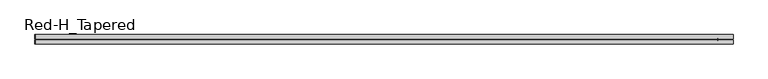
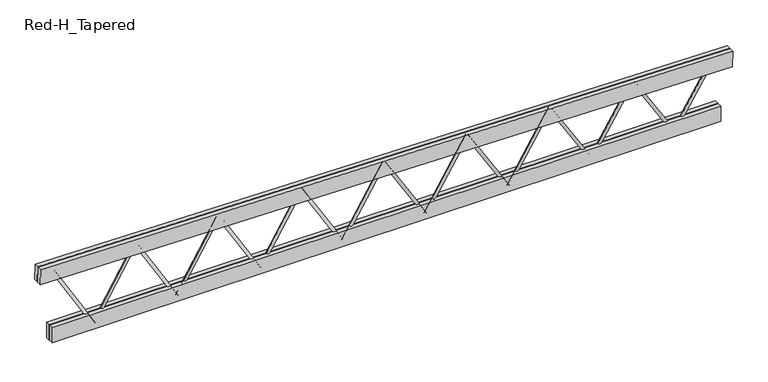
"""IFC4 building model written with IfcOpenShell, lengths in millimetres: beam geometry, Construction_Frames_RedBuilt_Openweb_Red-H_Tapered : Red-H_Tapered."""

from ifc_helpers import new_model, si_unit, point, frame, origin, origin_2d, place, context, project, spatial, polyline, circle_curve, trimmed, segment, composite_curve, outline, extrude, source, transform, mapped, element, save


def red_h_tapered_b0e51fd6(model_context):
    return source(origin(), model_context, "Body", "SweptSolid", [
        extrude(outline(composite_curve([segment(trimmed(circle_curve(origin_2d(), 12.7), [point((0.0, 12.7000001))], [point((0.0, -12.7))], False, "CARTESIAN"), True, "CONTINUOUS"), segment(trimmed(circle_curve(origin_2d(), 12.7), [point((0.0, -12.7))], [point((0.0, 12.7000001))], False, "CARTESIAN"), True, "CONTINUOUS")], self_intersect=False)), frame((2530.5740404, 0.0, -367.0101562), z_axis=(0.5262103953903533, 0.0, 0.8503544083399157), x_axis=(0.0, -1.0, 0.0)), (0.0, 0.0, 1.0), 687.0076691),
        extrude(outline(composite_curve([segment(trimmed(circle_curve(origin_2d(), 12.7), [point((0.0, -12.7))], [point((0.0, 12.7))], False, "CARTESIAN"), True, "CONTINUOUS"), segment(trimmed(circle_curve(origin_2d(), 12.7), [point((0.0, 12.7))], [point((0.0, -12.7))], False, "CARTESIAN"), True, "CONTINUOUS")], self_intersect=False)), frame((2530.5740404, 0.0, -367.0101562), z_axis=(-0.5236364879758304, 0.0, 0.8519417987517328), x_axis=(0.0, -1.0, 0.0)), (0.0, 0.0, 1.0), 690.3846189),
        extrude(outline(composite_curve([segment(trimmed(circle_curve(origin_2d(), 12.7), [point((0.0, 12.7))], [point((0.0, -12.6999999))], False, "CARTESIAN"), True, "CONTINUOUS"), segment(trimmed(circle_curve(origin_2d(), 12.7), [point((0.0, -12.6999999))], [point((0.0, 12.7))], False, "CARTESIAN"), True, "CONTINUOUS")], self_intersect=False)), frame((1807.552886, 0.0, -367.0101562), z_axis=(0.5236364879758294, 0.0, 0.8519417987517335), x_axis=(0.0, -1.0, 0.0)), (0.0, 0.0, 1.0), 690.3846189),
        extrude(outline(composite_curve([segment(trimmed(circle_curve(origin_2d(), 12.7), [point((0.0, -12.7))], [point((0.0, 12.7))], False, "CARTESIAN"), True, "CONTINUOUS"), segment(trimmed(circle_curve(origin_2d(), 12.7), [point((0.0, 12.7))], [point((0.0, -12.7))], False, "CARTESIAN"), True, "CONTINUOUS")], self_intersect=False)), frame((1807.552886, 0.0, -367.0101562), z_axis=(-0.5210829422122787, 0.0, 0.8535060441118124), x_axis=(0.0, -1.0, 0.0)), (0.0, 0.0, 1.0), 693.7678207),
        extrude(outline(composite_curve([segment(trimmed(circle_curve(origin_2d(), 12.7), [point((0.0, 12.7000001))], [point((0.0, -12.6999999))], False, "CARTESIAN"), True, "CONTINUOUS"), segment(trimmed(circle_curve(origin_2d(), 12.7), [point((0.0, -12.6999999))], [point((0.0, 12.7000001))], False, "CARTESIAN"), True, "CONTINUOUS")], self_intersect=False)), frame((1084.5317316, 0.0, -367.0101562), z_axis=(0.5210829422122776, 0.0, 0.8535060441118131), x_axis=(0.0, -1.0, 0.0)), (0.0, 0.0, 1.0), 693.7678207),
        extrude(outline(composite_curve([segment(trimmed(circle_curve(origin_2d(), 12.7), [point((0.0, -12.7))], [point((0.0, 12.7))], False, "CARTESIAN"), True, "CONTINUOUS"), segment(trimmed(circle_curve(origin_2d(), 12.7), [point((0.0, 12.7))], [point((0.0, -12.7))], False, "CARTESIAN"), True, "CONTINUOUS")], self_intersect=False)), frame((1084.5317316, 0.0, -367.0101562), z_axis=(-0.5185495980628914, 0.0, 0.855047550928493), x_axis=(0.0, -1.0, 0.0)), (0.0, 0.0, 1.0), 697.1571833),
        extrude(outline(composite_curve([segment(trimmed(circle_curve(origin_2d(), 12.7), [point((0.0, 12.7))], [point((0.0, -12.7))], False, "CARTESIAN"), True, "CONTINUOUS"), segment(trimmed(circle_curve(origin_2d(), 12.7), [point((0.0, -12.7))], [point((0.0, 12.7))], False, "CARTESIAN"), True, "CONTINUOUS")], self_intersect=False)), frame((361.5105772, 0.0, -367.0101562), z_axis=(0.5185495980628919, 0.0, 0.8550475509284927), x_axis=(0.0, -1.0, 0.0)), (0.0, 0.0, 1.0), 697.1571833),
        extrude(outline(composite_curve([segment(trimmed(circle_curve(origin_2d(), 12.7), [point((0.0, -12.7))], [point((0.0, 12.7))], False, "CARTESIAN"), True, "CONTINUOUS"), segment(trimmed(circle_curve(origin_2d(), 12.7), [point((0.0, 12.7))], [point((0.0, -12.7))], False, "CARTESIAN"), True, "CONTINUOUS")], self_intersect=False)), frame((361.5105772, 0.0, -367.0101562), z_axis=(-0.5160362950207581, 0.0, 0.8565667179042443), x_axis=(0.0, -1.0, 0.0)), (0.0, 0.0, 1.0), 700.5526175),
        extrude(outline(composite_curve([segment(trimmed(circle_curve(origin_2d(), 12.7), [point((0.0, -12.7))], [point((0.0, 12.7))], False, "CARTESIAN"), True, "CONTINUOUS"), segment(trimmed(circle_curve(origin_2d(), 12.7), [point((0.0, 12.7))], [point((0.0, -12.7))], False, "CARTESIAN"), True, "CONTINUOUS")], self_intersect=False)), frame((-361.5105772, 0.0, -367.0101562), z_axis=(0.5160362950207268, 0.0, 0.8565667179042632), x_axis=(0.0, -1.0, 0.0)), (0.0, 0.0, 1.0), 700.5526175),
        extrude(outline(composite_curve([segment(trimmed(circle_curve(origin_2d(), 12.7), [point((0.0, 12.7))], [point((0.0, -12.7))], False, "CARTESIAN"), True, "CONTINUOUS"), segment(trimmed(circle_curve(origin_2d(), 12.7), [point((0.0, -12.7))], [point((0.0, 12.7))], False, "CARTESIAN"), True, "CONTINUOUS")], self_intersect=False)), frame((-361.5105772, 0.0, -367.0101562), z_axis=(-0.5135428722107241, 0.0, 0.8580639360802667), x_axis=(0.0, -1.0, 0.0)), (0.0, 0.0, 1.0), 703.9540353),
        extrude(outline(composite_curve([segment(trimmed(circle_curve(origin_2d(), 12.7), [point((0.0, -12.7))], [point((0.0, 12.7))], False, "CARTESIAN"), True, "CONTINUOUS"), segment(trimmed(circle_curve(origin_2d(), 12.7), [point((0.0, 12.7))], [point((0.0, -12.7))], False, "CARTESIAN"), True, "CONTINUOUS")], self_intersect=False)), frame((-1084.5317316, 0.0, -367.0101562), z_axis=(0.5135428722107226, 0.0, 0.8580639360802675), x_axis=(0.0, -1.0, 0.0)), (0.0, 0.0, 1.0), 703.9540353),
        extrude(outline(composite_curve([segment(trimmed(circle_curve(origin_2d(), 12.7), [point((0.0, 12.7))], [point((0.0, -12.7))], False, "CARTESIAN"), True, "CONTINUOUS"), segment(trimmed(circle_curve(origin_2d(), 12.7), [point((0.0, -12.7))], [point((0.0, 12.7))], False, "CARTESIAN"), True, "CONTINUOUS")], self_intersect=False)), frame((-1084.5317316, 0.0, -367.0101562), z_axis=(-0.5110691684864845, 0.0, 0.8595395889792008), x_axis=(0.0, -1.0, 0.0)), (0.0, 0.0, 1.0), 707.3613505),
        extrude(outline(composite_curve([segment(trimmed(circle_curve(origin_2d(), 12.7), [point((0.0, -12.7))], [point((0.0, 12.7))], False, "CARTESIAN"), True, "CONTINUOUS"), segment(trimmed(circle_curve(origin_2d(), 12.7), [point((0.0, 12.7))], [point((0.0, -12.7))], False, "CARTESIAN"), True, "CONTINUOUS")], self_intersect=False)), frame((-1807.552886, 0.0, -367.0101562), z_axis=(0.5110691684864975, 0.0, 0.859539588979193), x_axis=(0.0, -1.0, 0.0)), (0.0, 0.0, 1.0), 707.3613505),
        extrude(outline(composite_curve([segment(trimmed(circle_curve(origin_2d(), 12.7), [point((0.0, 12.6999999))], [point((0.0, -12.7))], False, "CARTESIAN"), True, "CONTINUOUS"), segment(trimmed(circle_curve(origin_2d(), 12.7), [point((0.0, -12.7))], [point((0.0, 12.6999999))], False, "CARTESIAN"), True, "CONTINUOUS")], self_intersect=False)), frame((-1807.552886, 0.0, -367.0101562), z_axis=(-0.5086150225225358, 0.0, 0.8609940527462431), x_axis=(0.0, -1.0, 0.0)), (0.0, 0.0, 1.0), 710.7744781),
        extrude(outline(composite_curve([segment(trimmed(circle_curve(origin_2d(), 12.7), [point((0.0, -12.7))], [point((0.0, 12.6999999))], False, "CARTESIAN"), True, "CONTINUOUS"), segment(trimmed(circle_curve(origin_2d(), 12.7), [point((0.0, 12.6999999))], [point((0.0, -12.7))], False, "CARTESIAN"), True, "CONTINUOUS")], self_intersect=False)), frame((-2530.5740404, 0.0, -367.0101562), z_axis=(0.5086150225225242, 0.0, 0.86099405274625), x_axis=(0.0, -1.0, 0.0)), (0.0, 0.0, 1.0), 710.7744781),
        extrude(outline(composite_curve([segment(trimmed(circle_curve(origin_2d(), 12.7), [point((0.0, 12.6999999))], [point((0.0, -12.7000001))], False, "CARTESIAN"), True, "CONTINUOUS"), segment(trimmed(circle_curve(origin_2d(), 12.7), [point((0.0, -12.7000001))], [point((0.0, 12.6999999))], False, "CARTESIAN"), True, "CONTINUOUS")], self_intersect=False)), frame((-2530.5740404, 0.0, -367.0101562), z_axis=(-0.506180272901699, 0.0, 0.8624276962883101), x_axis=(0.0, -1.0, 0.0)), (0.0, 0.0, 1.0), 714.193335),
        extrude(outline(polyline([(-2917.4846176, -41.275), (-2917.4846176, -3.175), (2917.4846176, -3.175), (2917.4846176, -41.275), (-2917.4846176, -41.275)])), frame((0.0, 0.0, -386.0601562), z_axis=(0.0, 0.0, 1.0), x_axis=(1.0, 0.0, 0.0)), (0.0, 0.0, 1.0), 139.7),
        extrude(outline(polyline([(-2917.4846176, 3.175), (-2917.4846176, 41.275), (2917.4846176, 41.275), (2917.4846176, 3.175), (-2917.4846176, 3.175)])), frame((0.0, 0.0, -386.0601562), z_axis=(0.0, 0.0, 1.0), x_axis=(1.0, 0.0, 0.0)), (0.0, 0.0, 1.0), 139.7),
        extrude(outline(polyline([(0.0, -38.1), (0.0, 0.0), (6039.0239505, 0.0), (6039.0239505, -38.1), (0.0, -38.1)])), frame((-3021.434918, -3.175, 185.4596158), z_axis=(0.016823910756796456, 0.0, 0.9998584679977699), x_axis=(0.9998584679977699, 0.0, -0.016823910756796456)), (0.0, 0.0, 1.0), 139.7),
        extrude(outline(polyline([(0.0, -38.1), (0.0, 0.0), (6039.0239505, 0.0), (6039.0239505, -38.1), (0.0, -38.1)])), frame((-3021.434918, 41.275, 185.4596158), z_axis=(0.016823910756796456, 0.0, 0.9998584679977699), x_axis=(0.9998584679977699, 0.0, -0.016823910756796456)), (0.0, 0.0, 1.0), 139.7),
    ])


if __name__ == "__main__":
    model = new_model("IFC4")
    model_context = context("Model", 3, world=origin())
    ifc_project = project(units=[si_unit("LENGTHUNIT", "METRE", prefix="MILLI")], contexts=[model_context])
    site = spatial("IfcSite", under=ifc_project)
    building = spatial("IfcBuilding", under=site)
    placement = place(None, origin())
    red_h_tapered_shape = red_h_tapered_b0e51fd6(model_context)
    element("IfcBeam", 1, ObjectType="Construction_Frames_RedBuilt_Openweb_Red-H_Tapered : Red-H_Tapered", at=placement, inside=building, context=model_context, shape_type="MappedRepresentation", body=[
        mapped(red_h_tapered_shape, transform((0.0, 0.0, 0.0), x_axis=(1.0, 0.0, 0.0), y_axis=(0.0, 1.0, 0.0), z_axis=(0.0, 0.0, 1.0))),
    ])
    save(model, "model.ifc")

# Revit data of these elements
# Type "Construction_Frames_RedBuilt_Openweb_Red-H_Tapered : Red-H_Tapered"
#   Youtube clip = ""
#   Weight Net (Kg) = "0"
#   Webs = "Up to 2\" diameter tubular steel"
#   Uniformat II Description = ""
#   Uniformat II Code = ""
#   Uniclass 2015 Name = "Softwood trusses"
#   Uniclass 2015 Code = "Pr_20_85_90_81"
#   Uniclass 2.0 Description = "Structural Framing Systems"
#   Uniclass 2.0 Code = "SS-15-10-75"
#   Uniclass 1.4 Description = "Trusses"
#   Uniclass 1.4 Code = "L3523"
#   UNSPSC Code = "30103606"
#   Technical description = "http://www.redbuilt.com/reference/literature-and-other-resources"
#   Region South America = "None"
#   Region Oceania = "None"
#   Region North America = "US"
#   Region Middle East = "None"
#   Region Europe = "None"
#   Region Asia = "None"
#   Region Antarctica = "None"
#   Region Africa = "None"
#   QR code = "http://bimobject.com/redbuilt/product/redbuilt-0003"
#   Product url = "http://www.redbuilt.com/products/default.aspx?id=2"
#   Product group = "Wood Trusses"
#   Product family = "Construction"
#   Product data url = "https://bimobject.com/redbuilt/product/redbuilt-0003"
#   Product certification = ""
#   Product SKU = "redbuilt-0003"
#   Product Page URL = "http://www.redbuilt.com/commercial-systems/red-m-red-h-open-web-trusses"
#   Product Guid = "2c5793f2-6ffb-4665-b825-cf90c048e711"
#   Product Documentation Link = "http://www.redbuilt.com/documents/OW_Guide_2017_07_LowRes_wLinks.pdf"
#   OmniClass Description = "Wood Trusses"
#   OmniClass Code = "23-13 35 19 13 17"
#   NBS Reference Description = ""
#   NBS Reference Code = ""
#   Material secondary = "Steel"
#   Material main = "CHARRED WOOD"
#   Masterformat 2014 Description = "Metal-Web Wood Joists"
#   Masterformat 2014 Code = "06 17 36"
#   Manufacturer name = "RedBuilt"
#   Manufacturer country = "United States"
#   Installation instructions = "http://www.redbuilt.com/documents/Installation_Sheets_Open-Web.pdf"
#   IFC Classification = ""
#   EAN code = ""
#   Design country = "United States"
#   Product Information = "http://redbuilt.com/products/default.aspx?id=2"
#   Model = "Red-H-Tapered"
#   Manufacturer URL = "http://redbuilt.com/"
#   Manufacturer = "RedBuilt™"
#   Description = "Open Web Truss"
#   Date of publishing = "8/17/2010"
#   Contact us = "http://redbuilt.com/contact/"
#   Chords = "Double 1½\" x 5½\" MSR lumber"
#   COBIe Type Category = ""
#   Brand url = "http://www.redbuilt.com"
#   BIMobject main category code = "construction"
#   BIMobject main category = "Construction"
#   BIMobject category code = "construction-frames-trusses"
#   BIMobject category = "Frames & Trusses"
#   Web Radius = 0' - 0 1/2"
#   Web Layout Offset Start [instance default] = 0' - 5"
#   Web Layout Offset End [instance default] = 0' - 5"
#   Web Diameter = 0' - 1"
#   TotalLength [instance default] = 20' - 0"
#   Span Minimum = 4' - 0"
#   Span Maximum = 70' - 0"
#   Span Limit [instance default] = 20' - 0"
#   Nominal width = 0' - 0"
#   Nominal height = 0' - 0"
#   Inner Depth Top [instance default] = 0' - 2.76372"
#   Depth Start [instance default] = 6' - 0"
#   Top Chord Length [instance default] = 20' - 1.19701"
#   TC Extension Start Aux [instance default] = 0' - 0"
#   TC Extension End Aux [instance default] = 0' - 0"
#   T-B Chord Length Difference L [instance default] = 0' - 4"
#   T-B Chord Length Difference [instance default] = 0' - 4"
#   Height 2 [instance default] = 6' - 0"
#   Depth Minimum at Wall = 2' - 0"
#   Depth Maximum at Wall = 6' - 0"
#   Depth Lower End [instance default] = 2' - 0"
#   Depth Higher End [instance default] = 6' - 0"
#   Depth End [instance default] = 2' - 0"
#   Depth 2 [instance default] = 2' - 0"
#   Chord Width = 0' - 3 1/4"
#   Chord Thickness = 0' - 1 1/2"
#   Chord Depth = 0' - 5 1/2"
#   Offset Start [instance default] = 0' - 0"
#   TC Extension Start [instance default] = 0' - 0"
#   End Panel = 0' - 5"
#   Offset End [instance default] = 0' - 0"
#   TC Extension End [instance default] = 0' - 0"
#   Length [instance default] = 20' - 0"
#   Angle [instance default] = 5.71059°
#   Span Limit Warning [instance default] = no
#   Edition number = 1
#   Top Bearing Start [instance default] = yes
#   Top Bearing End [instance default] = yes
#   Bottom Bearing Start [instance default] = no
#   Bottom Bearing End [instance default] = no
#   8 Panels [instance default] = yes
#   16 Panels [instance default] = no
#   12 Panels [instance default] = no
#   Web Material = RedBuilt-Steel, Galvanized
#   Clip Material = RedBuilt-Steel, Galvanized
#   Chords Material = WOOD-OAKFIRE
#   URL = ""
#   Assembly Code = ""
# Element 1 (IfcBeam, "Construction_Frames_RedBuilt_Openweb_Red-H_Tapered : Red-H_Tapered")
#   TotalLength = 19' - 9.7232"
#   Span Limit = 19' - 9.7232"
#   Inner Depth Top = 0' - 2.75039"
#   Depth Start = 5' - 0"
#   Top Chord Length = 19' - 9.75685"
#   Height 2 = 5' - 0"
#   Depth Higher End = 5' - 0"
#   Depth 2 = 0' - 4"
#   Angle = 0.963985°
#   Materials on its faces: "RedBuilt-Steel, Galvanized", "WOOD-OAKFIRE"
# Materials
#   "RedBuilt-Steel, Galvanized": class "Metal", colour RGB 164 172 176, transparency 0, Manufacturer = "RedBuilt. LLC", Comments = "Openweb Metal Web", URL = "http://www.redbuilt.com/", Description = "Galvanized steel", Cost = 0
#   "WOOD-OAKFIRE": class "Wood", colour RGB 198 202 183, transparency 0, Description = "Generic wood", Cost = 0
